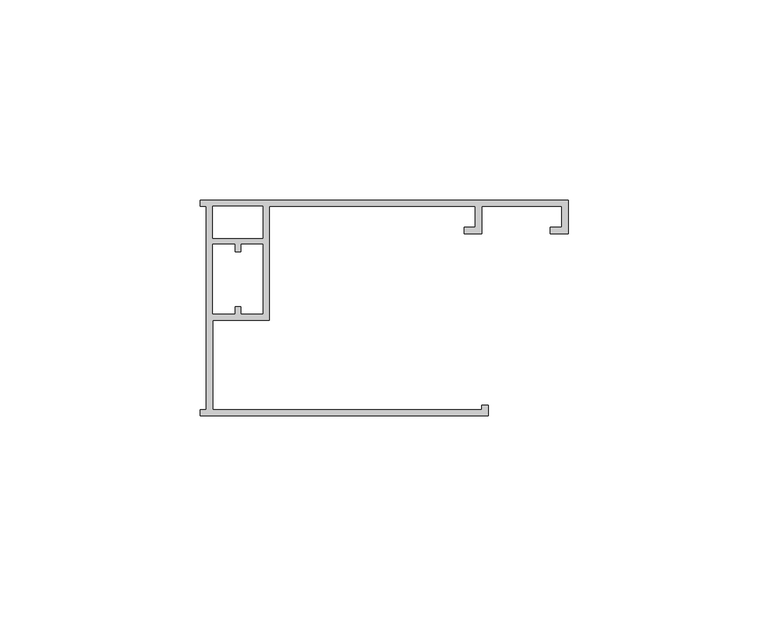
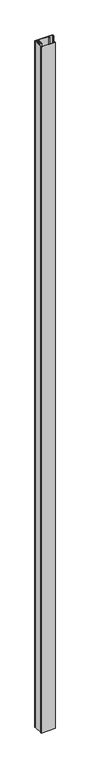
"""IFC4 building model written with IfcOpenShell, lengths in millimetres: proxy geometry, Generic Models 2:Generic Models 2:310765:Generic Models 2:310765 : Generic Models 2:Generic Models 2:310765:55 : Generic Models 2:Generic Models 2:310765:Generic Models 2:310765 : Generic Models 2:Generic Models 2:310765:300385."""

from ifc_helpers import new_model, si_unit, frame, origin, place, context, project, spatial, polyline, outline, extrude, source, transform, mapped, element, save


def generic_models_7ecf8543(model_context):
    return source(origin(), model_context, "Body", "SweptSolid", [
        extrude(outline(polyline([(578590.1363239, -568270.7619958), (578591.7238239, -568270.7619958), (578591.7238239, -568219.9369958), (578590.1363239, -568219.9369958), (578590.1363239, -568218.3494958), (578682.1363239, -568218.3494958), (578682.1363239, -568226.7958673), (578677.7489974, -568226.7958673), (578677.7489974, -568225.2083673), (578680.5488239, -568225.2083673), (578680.5488239, -568219.9369958), (578660.5488239, -568219.9369958), (578660.5488239, -568226.7958673), (578656.1614974, -568226.7958673), (578656.1614974, -568225.2083673), (578658.9613239, -568225.2083673), (578658.9613239, -568219.9369958), (578607.4688212, -568219.9369958), (578607.4688212, -568248.401137), (578593.3113239, -568248.401137), (578593.3113239, -568270.7619958), (578660.5488239, -568270.7619958), (578660.5488239, -568269.6344059), (578662.1363239, -568269.6344059), (578662.1363239, -568272.3494958), (578590.1363239, -568272.3494958), (578590.1363239, -568270.7619958)]), holes=[polyline([(578593.3113239, -568246.813637), (578598.8025726, -568246.813637), (578598.8025726, -568244.8882215), (578600.3900726, -568244.8882215), (578600.3900726, -568246.813637), (578605.8813212, -568246.813637), (578605.8813212, -568229.4676308), (578600.3900726, -568229.4676308), (578600.3900726, -568231.3930462), (578598.8025726, -568231.3930462), (578598.8025726, -568229.4676308), (578593.3113239, -568229.4676308), (578593.3113239, -568246.813637)]), polyline([(578605.8813212, -568219.9369958), (578593.3113239, -568219.9369958), (578593.3113239, -568227.8801308), (578605.8813212, -568227.8801308), (578605.8813212, -568219.9369958)])]), frame((0.0, 0.0, 4860.0679991), z_axis=(0.0, 0.0, 1.0), x_axis=(1.0, 0.0, 0.0)), (0.0, 0.0, 1.0), 3695.7),
    ])


if __name__ == "__main__":
    model = new_model("IFC4")
    model_context = context("Model", 3, world=origin())
    ifc_project = project(units=[si_unit("LENGTHUNIT", "METRE", prefix="MILLI")], contexts=[model_context])
    site = spatial("IfcSite", under=ifc_project)
    building = spatial("IfcBuilding", under=site)
    placement = place(None, origin())
    generic_models_shape = generic_models_7ecf8543(model_context)
    element("IfcBuildingElementProxy", 1, Name="Generic Models 2:Generic Models 2:310765:Generic Models 2:310765 : Generic Models 2:Generic Models 2:310765:55 : Generic Models 2:Generic Models 2:310765:Generic Models 2:310765 : Generic Models 2:Generic Models 2:310765:300385", ObjectType="Generic Models 2:Generic Models 2:310765:Generic Models 2:310765 : Generic Models 2:Generic Models 2:310765:55 : Generic Models 2:Generic Models 2:310765:Generic Models 2:310765 : Generic Models 2:Generic Models 2:310765:300385", at=placement, inside=building, context=model_context, shape_type="MappedRepresentation", body=[
        mapped(generic_models_shape, transform((0.0, 0.0, 0.0), x_axis=(1.0, 0.0, 0.0), y_axis=(0.0, 1.0, 0.0), z_axis=(0.0, 0.0, 1.0))),
    ])
    save(model, "model.ifc")

# Revit data of these elements
# Type "Generic Models 2:Generic Models 2:310765:Generic Models 2:310765 : Generic Models 2:Generic Models 2:310765:55 : Generic Models 2:Generic Models 2:310765:Generic Models 2:310765 : Generic Models 2:Generic Models 2:310765:300385"
#   NameOverride = "Generic Models 2:Generic Models 2:310765:Generic Models 2:310765 : Generic Models 2:Generic Models 2:310765:300385"
#   ObjectTypeOverride = "Generic Models 2:310765 : Generic Models 2:Generic Models 2:310765"
#   Reference = "Generic Models 2"
#   Tag = "300385"
# Element 1 (IfcBuildingElementProxy, "Generic Models 2:Generic Models 2:310765:Generic Models 2:310765 : Generic Models 2:Generic Models 2:310765:55 : Generic Models 2:Generic Models 2:310765:Generic Models 2:310765 : Generic Models 2:Generic Models 2:310765:300385")
#   Materials on its faces: "THERMAL BROKEN ALUMINUM STOREFRONT FOR POLYCARBONATE"
# Materials
#   "THERMAL BROKEN ALUMINUM STOREFRONT FOR POLYCARBONATE": class "Unassigned", colour RGB 244 244 244, transparency 0, Keynote = "M07611300.01", Cost = 0
